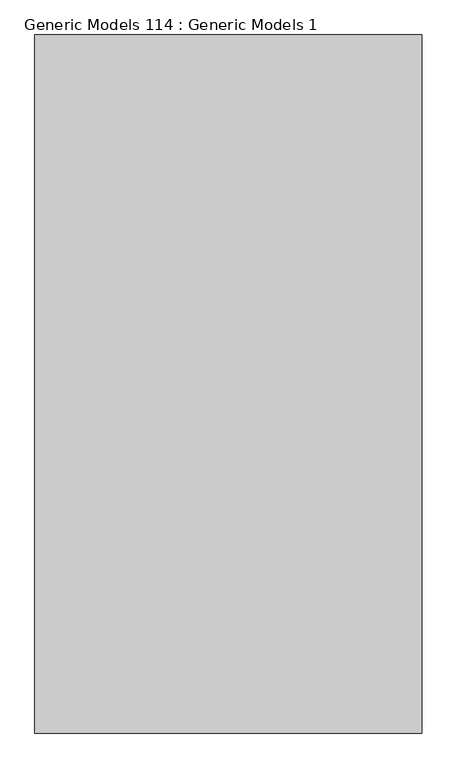
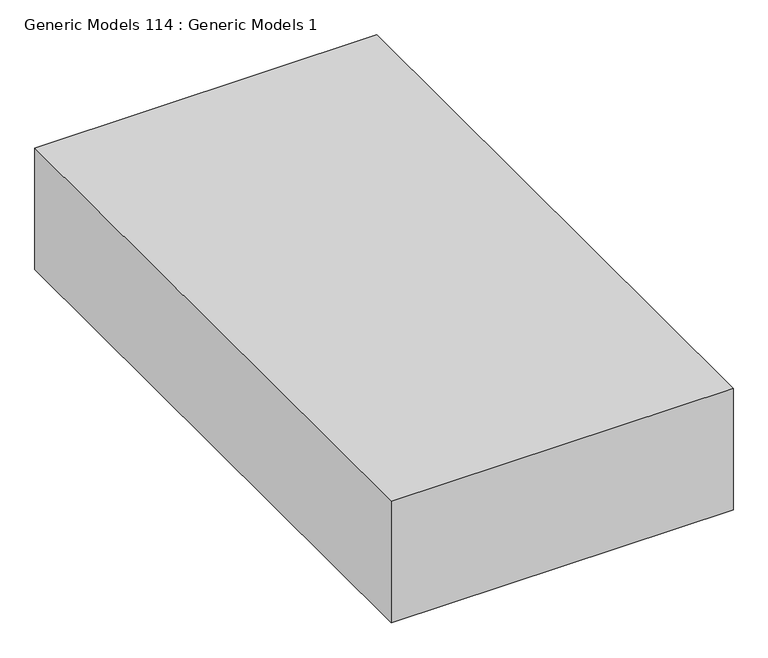
"""IFC4 building model written with IfcOpenShell, lengths in millimetres: proxy geometry, Generic Models 114 : Generic Models 1."""

import ifcopenshell
import ifcopenshell.guid

model = None  # the IFC model being written
_history = None  # IfcOwnerHistory: only IFC2X3 demands one
_inside = {}  # id of a spatial element -> (the spatial element, [elements in it])
_under = {}  # id of a project, library or spatial element -> (it, [spatial elements below it])
_declared = {}  # id of a project -> (the project, [libraries it declares])
_typed = {}  # id of a type object -> (the type object, [elements of that type])
_made_of = {}  # id of a material, layer set ... -> (it, [elements and type objects made of it])


def new_model(schema):
    """Start an empty IFC model of exactly this schema.

    Asked for "IFC4X3", IfcOpenShell would pick the latest addendum, in which some entities
    have other attributes; the version numbers below select the first issue.
    IFC2X3 requires an IfcOwnerHistory on every rooted entity: one is made here for all.
    """
    global model, _history
    if schema == "IFC4X3":
        model = ifcopenshell.file(schema_version=(4, 3, 0, 0))
    else:
        model = ifcopenshell.file(schema=schema)
    _inside.clear()
    _under.clear()
    _declared.clear()
    _typed.clear()
    _made_of.clear()
    _history = None
    if model.schema == "IFC2X3":
        org = make("IfcOrganization", Name="unknown")
        user = make(
            "IfcPersonAndOrganization",
            ThePerson=make("IfcPerson", FamilyName="unknown"),
            TheOrganization=org,
        )
        app = make(
            "IfcApplication",
            ApplicationDeveloper=org,
            Version="unknown",
            ApplicationFullName="unknown",
            ApplicationIdentifier="unknown",
        )
        _history = make(
            "IfcOwnerHistory",
            OwningUser=user,
            OwningApplication=app,
            ChangeAction="ADDED",
            CreationDate=0,
        )
    return model


def make(cls, **values):
    """One entity of the class cls with the attributes given. An attribute that is None is left unset."""
    return model.create_entity(
        cls, **{name: value for name, value in values.items() if value is not None}
    )


def rooted(cls, **values):
    """An entity with a GlobalId (a new one), such as an element, a storey or a relation."""
    return make(cls, GlobalId=ifcopenshell.guid.new(), OwnerHistory=_history, **values)


def si_unit(unit_type, name, prefix=None):
    """IfcSIUnit, for example si_unit("LENGTHUNIT", "METRE", prefix="MILLI")."""
    return make("IfcSIUnit", UnitType=unit_type, Prefix=prefix, Name=name)


def assignment(units):
    """IfcUnitAssignment: the units of a project."""
    return None if units is None else make("IfcUnitAssignment", Units=units)


def point(xyz):
    """IfcCartesianPoint."""
    return None if xyz is None else make("IfcCartesianPoint", Coordinates=xyz)


def direction(xyz):
    """IfcDirection."""
    return None if xyz is None else make("IfcDirection", DirectionRatios=xyz)


def frame(location, z_axis=None, x_axis=None):
    """IfcAxis2Placement3D, a coordinate frame: its origin and axes. An axis left out is left unset."""
    return make(
        "IfcAxis2Placement3D",
        Location=point(location),
        Axis=direction(z_axis),
        RefDirection=direction(x_axis),
    )


def origin():
    """The frame at (0, 0, 0) with its axes left unset."""
    return frame((0.0, 0.0, 0.0))


def place(relative_to, where):
    """IfcLocalPlacement: puts the frame where relative to a parent placement (None: the world)."""
    return make(
        "IfcLocalPlacement", PlacementRelTo=relative_to, RelativePlacement=where
    )


def context(
    kind, dimensions, precision=None, world=None, true_north=None, identifier=None
):
    """IfcGeometricRepresentationContext, for example the 3D "Model" context."""
    return make(
        "IfcGeometricRepresentationContext",
        ContextIdentifier=identifier,
        ContextType=kind,
        CoordinateSpaceDimension=dimensions,
        Precision=precision,
        WorldCoordinateSystem=world,
        TrueNorth=true_north,
    )


def project(units=None, contexts=None):
    """IfcProject with its units and contexts."""
    return rooted(
        "IfcProject",
        Name="project",
        RepresentationContexts=contexts,
        UnitsInContext=assignment(units),
    )


def spatial(cls, under=None, at=None, **own):
    """A site, building, storey or space (cls), placed at a placement, below another one or the project."""
    s = rooted(cls, ObjectPlacement=at, **own)
    if under is not None:
        _under.setdefault(under.id(), (under, []))[1].append(s)
    return s


def polyline(points):
    """IfcPolyline through the points."""
    return make("IfcPolyline", Points=[point(p) for p in points])


def outline(outer, holes=None, kind="AREA"):
    """IfcArbitraryClosedProfileDef: a profile drawn as a closed curve; with holes, ...WithVoids."""
    if holes is None:
        return make("IfcArbitraryClosedProfileDef", ProfileType=kind, OuterCurve=outer)
    return make(
        "IfcArbitraryProfileDefWithVoids",
        ProfileType=kind,
        OuterCurve=outer,
        InnerCurves=holes,
    )


def extrude(swept, where, along, depth):
    """IfcExtrudedAreaSolid: the profile swept, set in the frame where, extruded along a direction by depth."""
    return make(
        "IfcExtrudedAreaSolid",
        SweptArea=swept,
        Position=where,
        ExtrudedDirection=direction(along),
        Depth=depth,
    )


def shape(context_of_items, identifier, shape_type, items):
    """IfcShapeRepresentation: the items that make up one representation, for example the "Body"."""
    return make(
        "IfcShapeRepresentation",
        ContextOfItems=context_of_items,
        RepresentationIdentifier=identifier,
        RepresentationType=shape_type,
        Items=items,
    )


def source(mapping_origin, context_of_items, identifier, shape_type, items):
    """IfcRepresentationMap: a shape defined once, which mapped items show again and again."""
    return make(
        "IfcRepresentationMap",
        MappingOrigin=mapping_origin,
        MappedRepresentation=shape(context_of_items, identifier, shape_type, items),
    )


def transform(
    local_origin,
    x_axis=None,
    y_axis=None,
    z_axis=None,
    scale=None,
    scale2=None,
    scale3=None,
    uniform=True,
):
    """IfcCartesianTransformationOperator3D, or its non-uniform kind. x_axis, y_axis, z_axis: its Axis1, 2, 3."""
    if uniform:
        return make(
            "IfcCartesianTransformationOperator3D",
            Axis1=direction(x_axis),
            Axis2=direction(y_axis),
            LocalOrigin=point(local_origin),
            Scale=scale,
            Axis3=direction(z_axis),
        )
    return make(
        "IfcCartesianTransformationOperator3DnonUniform",
        Axis1=direction(x_axis),
        Axis2=direction(y_axis),
        LocalOrigin=point(local_origin),
        Scale=scale,
        Axis3=direction(z_axis),
        Scale2=scale2,
        Scale3=scale3,
    )


def mapped(mapping_source, mapping_target):
    """IfcMappedItem: shows the shape of a source again, moved by a transform."""
    return make(
        "IfcMappedItem", MappingSource=mapping_source, MappingTarget=mapping_target
    )


def made_of(thing, what):
    """Note that an element or type object is made of a material, layer set ...; save() writes the relation."""
    if what is not None:
        _made_of.setdefault(what.id(), (what, []))[1].append(thing)
    return thing


def element(
    cls,
    number,
    at=None,
    inside=None,
    cuts=None,
    type_object=None,
    material=None,
    context=None,
    identifier="Body",
    shape_type=None,
    held_by="IfcProductDefinitionShape",
    body=None,
    shapes=None,
    **own,
):
    """One element of the class cls, such as IfcWall. Its Tag is "e" and its number.

    at: its placement. inside: the storey or other place that contains it. cuts: it is an
    opening in that element (IfcRelVoidsElement). A single representation is given by context,
    identifier, shape_type and body (its items); several are given by shapes. held_by: the class
    of the entity that holds the representations. save() writes the other relations.
    """
    e = rooted(cls, Tag="e%d" % number, ObjectPlacement=at, **own)
    if body is not None:
        shapes = [shape(context, identifier, shape_type, body)]
    if shapes is not None:
        e.Representation = make(held_by, Representations=shapes)
    if inside is not None:
        _inside.setdefault(inside.id(), (inside, []))[1].append(e)
    if cuts is not None:
        rooted(
            "IfcRelVoidsElement", RelatingBuildingElement=cuts, RelatedOpeningElement=e
        )
    if type_object is not None:
        _typed.setdefault(type_object.id(), (type_object, []))[1].append(e)
    return made_of(e, material)


def aggregate(whole, parts):
    """IfcRelAggregates: a whole, such as a stair, and the parts it consists of."""
    return rooted("IfcRelAggregates", RelatingObject=whole, RelatedObjects=parts)


def save(model, path):
    """Write the relations noted so far, then the file.

    IfcRelAggregates (storeys below a building ...), IfcRelContainedInSpatialStructure (elements
    in a storey), IfcRelDefinesByType, IfcRelAssociatesMaterial and IfcRelDeclares: one each for
    every whole, place, type object, material and project.
    """
    for whole, parts in _under.values():
        aggregate(whole, parts)
    for where, things in _inside.values():
        rooted(
            "IfcRelContainedInSpatialStructure",
            RelatedElements=things,
            RelatingStructure=where,
        )
    for kind, things in _typed.values():
        rooted("IfcRelDefinesByType", RelatedObjects=things, RelatingType=kind)
    for what, things in _made_of.values():
        rooted("IfcRelAssociatesMaterial", RelatedObjects=things, RelatingMaterial=what)
    for by, libraries in _declared.values():
        rooted("IfcRelDeclares", RelatingContext=by, RelatedDefinitions=libraries)
    model.write(path)


def generic_models_114_generic_models_1_a6fb1c2c(model_context):
    return source(origin(), model_context, "Body", "SweptSolid", [
        extrude(outline(polyline([(51642.1451407, 1219.2), (51642.1451407, 0.0), (50965.9242022, 0.0), (50965.9242022, 1219.2), (51642.1451407, 1219.2)])), frame((0.0, 0.0, 5237.6235034), z_axis=(0.0, 0.0, 1.0), x_axis=(1.0, 0.0, 0.0)), (0.0, 0.0, 1.0), 254.0),
    ])


if __name__ == "__main__":
    model = new_model("IFC4")
    model_context = context("Model", 3, world=origin())
    ifc_project = project(units=[si_unit("LENGTHUNIT", "METRE", prefix="MILLI")], contexts=[model_context])
    site = spatial("IfcSite", under=ifc_project)
    building = spatial("IfcBuilding", under=site)
    placement = place(None, origin())
    generic_models_114_generic_models_1_shape = generic_models_114_generic_models_1_a6fb1c2c(model_context)
    element("IfcBuildingElementProxy", 1, Name="Generic Models 114 : Generic Models 1", ObjectType="Generic Models 114 : Generic Models 1", at=placement, inside=building, context=model_context, shape_type="MappedRepresentation", body=[
        mapped(generic_models_114_generic_models_1_shape, transform((0.0, 0.0, 0.0), x_axis=(1.0, 0.0, 0.0), y_axis=(0.0, 1.0, 0.0), z_axis=(0.0, 0.0, 1.0))),
    ])
    save(model, "model.ifc")

# Revit data of these elements
# Element 1 (IfcBuildingElementProxy, "Generic Models 114 : Generic Models 1")
#   Materials on its faces: "SOUND BATT. INSULATION"
# Materials
#   "SOUND BATT. INSULATION": class "Unassigned", colour RGB 255 255 255, transparency 0, Cost = 0
